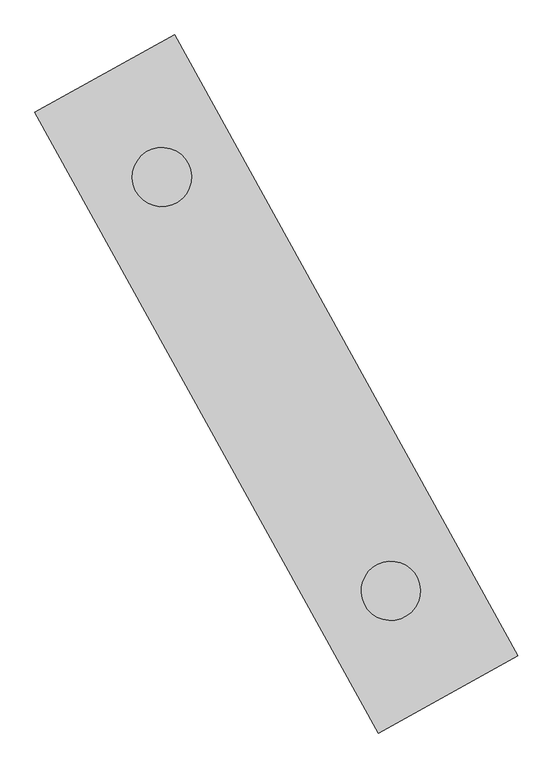
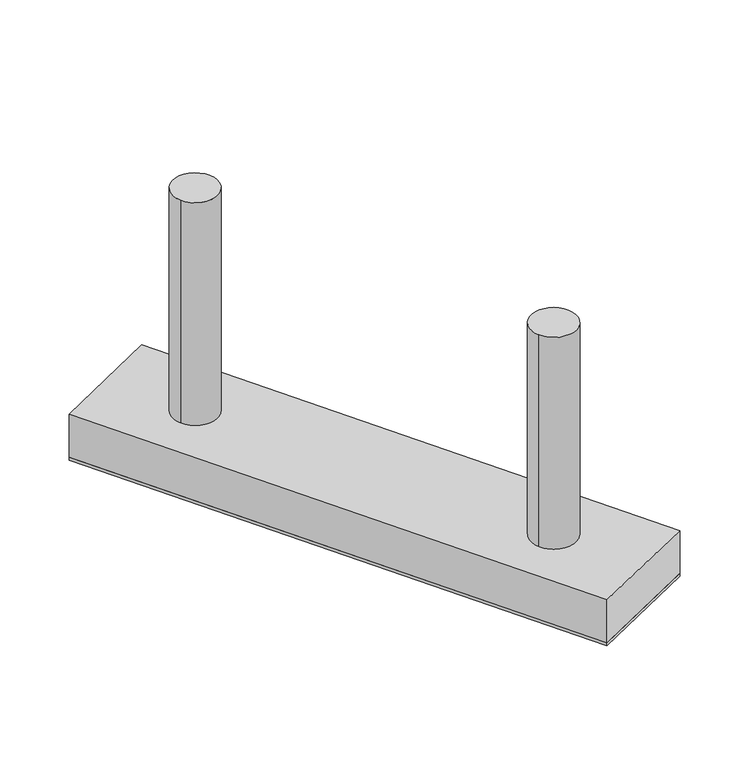
"""IFC4 building model written with IfcOpenShell, lengths in millimetres: beam geometry, KNA_SF_TSP as3 : KNA_SF_TSP as3."""

from ifc_helpers import new_model, si_unit, point, frame, frame_2d, origin, place, context, project, spatial, polyline, circle_curve, trimmed, segment, composite_curve, outline, extrude, source, transform, mapped, element, save


def beam_fb94c7fa(model_context):
    return source(origin(), model_context, "Body", "SweptSolid", [
        extrude(outline(composite_curve([segment(trimmed(circle_curve(frame_2d((156804.6150839, -36190.7589555)), 500.0), [point((156355.4073342, -36410.3321723))], [point((157253.8228337, -35971.1857387))], False, "CARTESIAN"), True, "CONTINUOUS"), segment(trimmed(circle_curve(frame_2d((156804.6150839, -36190.7589555)), 500.0), [point((157253.8228337, -35971.1857387))], [point((156355.4073342, -36410.3321723))], False, "CARTESIAN"), True, "CONTINUOUS")], self_intersect=False)), frame((0.0, 0.0, -1600.0), z_axis=(0.0, 0.0, 1.0), x_axis=(1.0, 0.0, 0.0)), (0.0, 0.0, 1.0), 4940.9999053),
        extrude(outline(composite_curve([segment(trimmed(circle_curve(frame_2d((152929.8715235, -29191.7331418)), 500.0), [point((152480.6637737, -29411.3063586))], [point((153379.0792733, -28972.159925))], False, "CARTESIAN"), True, "CONTINUOUS"), segment(trimmed(circle_curve(frame_2d((152929.8715235, -29191.7331418)), 500.0), [point((153379.0792733, -28972.159925))], [point((152480.6637737, -29411.3063586))], False, "CARTESIAN"), True, "CONTINUOUS")], self_intersect=False)), frame((0.0, 0.0, -1600.0), z_axis=(0.0, 0.0, 1.0), x_axis=(1.0, 0.0, 0.0)), (0.0, 0.0, 1.0), 5194.9321792),
        extrude(outline(polyline([(156592.215368, -38594.3783848), (150780.1000273, -28095.8396642), (153142.2712395, -26788.1137126), (158954.3865801, -37286.6524331), (156592.215368, -38594.3783848)])), frame((0.0, 0.0, -2600.0), z_axis=(0.0, 0.0, 1.0), x_axis=(1.0, 0.0, 0.0)), (0.0, 0.0, 1.0), 1000.0),
        extrude(outline(polyline([(150780.1000273, -28095.8396642), (153142.2712395, -26788.1137126), (158954.3865801, -37286.6524331), (156592.215368, -38594.3783848), (150780.1000273, -28095.8396642)])), frame((0.0, 0.0, -2670.0), z_axis=(0.0, 0.0, 1.0), x_axis=(1.0, 0.0, 0.0)), (0.0, 0.0, 1.0), 70.0),
    ])


if __name__ == "__main__":
    model = new_model("IFC4")
    model_context = context("Model", 3, world=origin())
    ifc_project = project(units=[si_unit("LENGTHUNIT", "METRE", prefix="MILLI")], contexts=[model_context])
    site = spatial("IfcSite", under=ifc_project)
    building = spatial("IfcBuilding", under=site)
    placement = place(None, origin())
    beam_shape = beam_fb94c7fa(model_context)
    element("IfcBeam", 1, ObjectType="KNA_SF_TSP as3 : KNA_SF_TSP as3", at=placement, inside=building, context=model_context, shape_type="MappedRepresentation", body=[
        mapped(beam_shape, transform((0.0, 0.0, 0.0), x_axis=(1.0, 0.0, 0.0), y_axis=(0.0, 1.0, 0.0), z_axis=(0.0, 0.0, 1.0))),
    ])
    save(model, "model.ifc")

# Revit data of these elements
# Element 1 (IfcBeam, "KNA_SF_TSP as3 : KNA_SF_TSP as3")
#   Materials on its faces: "Beton_Bestaande Constructie", "Beton_In-Situ_Werkvloer"
# Materials
#   "Beton_Bestaande Constructie": class "Concrete", colour RGB 102 102 102, transparency 0, Description = "Beton", Cost = 0
#   "Beton_In-Situ_Werkvloer": class "Concrete", colour RGB 128 128 128, transparency 0, Description = "Beton", Cost = 0
